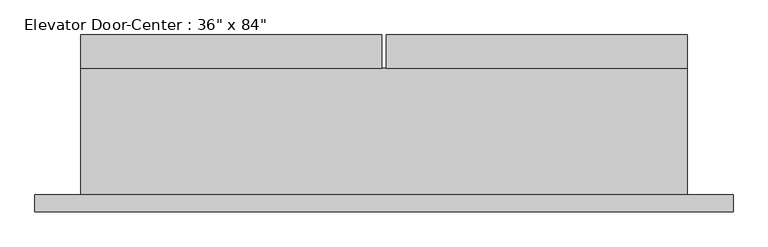
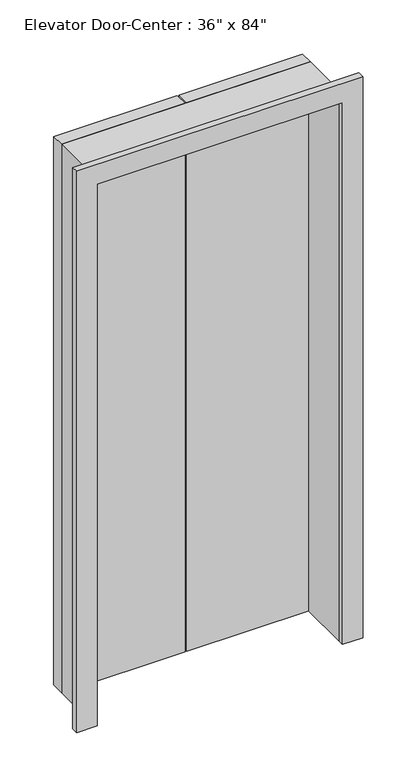
"""IFC4 building model written with IfcOpenShell, lengths in millimetres: proxy geometry."""

from ifc_helpers import new_model, si_unit, frame, origin, origin_with_axes, place, context, project, spatial, polyline, outline, extrude, source, transform, mapped, element, save


def proxy_71d7088b(model_context):
    return source(origin(), model_context, "Body", "SweptSolid", [
        extrude(outline(polyline([(-102.3106443, 96.8375), (-562.6856443, 96.8375), (-562.6856443, 147.6375), (-102.3106443, 147.6375), (-102.3106443, 96.8375)])), origin_with_axes(), (0.0, 0.0, 1.0), 2159.0),
        extrude(outline(polyline([(364.4143557, 96.8375), (-95.9606443, 96.8375), (-95.9606443, 147.6375), (364.4143557, 147.6375), (364.4143557, 96.8375)])), origin_with_axes(), (0.0, 0.0, 1.0), 2159.0),
        extrude(outline(polyline([(0.0, -562.6856443), (0.0, -556.3356443), (2133.6, -556.3356443), (2133.6, 358.0643557), (0.0, 358.0643557), (0.0, 364.4143557), (2159.0, 364.4143557), (2159.0, -562.6856443), (0.0, -562.6856443)])), frame((0.0, -96.8375, 0.0), z_axis=(0.0, 1.0, 0.0), x_axis=(0.0, 0.0, 1.0)), (0.0, 0.0, 1.0), 193.675),
        extrude(outline(polyline([(0.0, -632.5356443), (0.0, -556.3356443), (2133.6, -556.3356443), (2133.6, 358.0643557), (0.0, 358.0643557), (0.0, 434.2643557), (2209.8, 434.2643557), (2209.8, -632.5356443), (0.0, -632.5356443)])), frame((0.0, -122.2375, 0.0), z_axis=(0.0, 1.0, 0.0), x_axis=(0.0, 0.0, 1.0)), (0.0, 0.0, 1.0), 25.4),
    ])


if __name__ == "__main__":
    model = new_model("IFC4")
    model_context = context("Model", 3, world=origin())
    ifc_project = project(units=[si_unit("LENGTHUNIT", "METRE", prefix="MILLI")], contexts=[model_context])
    site = spatial("IfcSite", under=ifc_project)
    building = spatial("IfcBuilding", under=site)
    placement = place(None, origin())
    proxy_shape = proxy_71d7088b(model_context)
    element("IfcBuildingElementProxy", 1, Name="Elevator Door-Center : 36\" x 84\"", ObjectType="Elevator Door-Center : 36\" x 84\"", at=placement, inside=building, context=model_context, shape_type="MappedRepresentation", body=[
        mapped(proxy_shape, transform((0.0, 0.0, 0.0), x_axis=(1.0, 0.0, 0.0), y_axis=(0.0, 1.0, 0.0), z_axis=(0.0, 0.0, 1.0))),
    ])
    save(model, "model.ifc")

# Revit data of these elements
# Type "Elevator Door-Center : 36\" x 84\""
#   Assembly Code = "D1010"
#   Door Height = 7' - 0"
#   Door Width = 3' - 0"
#   Trim Projection = 0' - 1"
#   Trim Width = 0' - 3"
#   Door Finish = Elevator Door
#   Frame Finish = Door - Frame
#   Default Elevation = 0
# Element 1 (IfcBuildingElementProxy, "Elevator Door-Center : 36\" x 84\"")
#   Materials on its faces: "Door - Frame", "Elevator Door"
# Materials
#   "Elevator Door": class "Metal", colour RGB 57 57 57, transparency 0
#   "Door - Frame": class "Miscellaneous", colour RGB 118 70 51, transparency 0, Cost = 0
